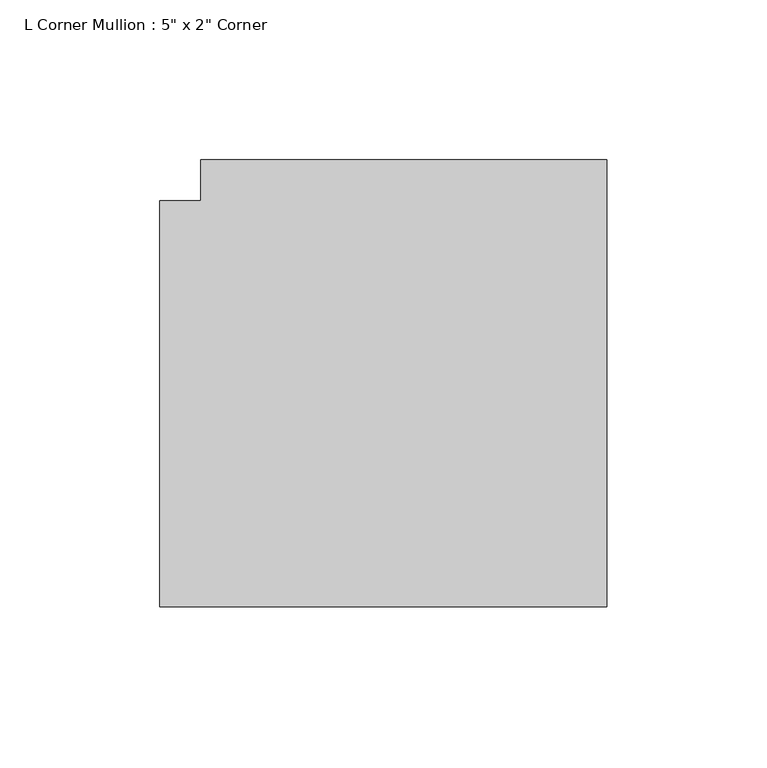
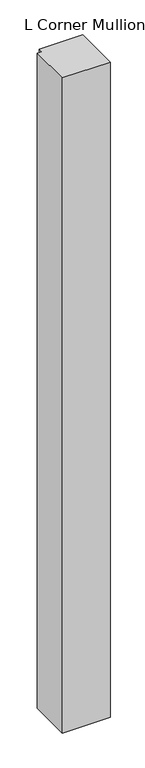
"""IFC4 building model written with IfcOpenShell, lengths in millimetres: member geometry."""

from ifc_helpers import new_model, si_unit, frame, origin, place, context, project, spatial, polyline, outline, extrude, source, transform, mapped, element, save


def member_8e92f094(model_context):
    return source(origin(), model_context, "Body", "SweptSolid", [
        extrude(outline(polyline([(63.5, 76.2), (63.5, -63.5), (-76.2, -63.5), (-76.2, 63.5), (-63.5, 63.5), (-63.5, 76.2), (63.5, 76.2)])), frame((0.0, 0.0, -2032.0), z_axis=(0.0, 0.0, 1.0), x_axis=(1.0, 0.0, 0.0)), (0.0, 0.0, 1.0), 2032.0),
    ])


if __name__ == "__main__":
    model = new_model("IFC4")
    model_context = context("Model", 3, world=origin())
    ifc_project = project(units=[si_unit("LENGTHUNIT", "METRE", prefix="MILLI")], contexts=[model_context])
    site = spatial("IfcSite", under=ifc_project)
    building = spatial("IfcBuilding", under=site)
    placement = place(None, origin())
    member_shape = member_8e92f094(model_context)
    element("IfcMember", 1, ObjectType="L Corner Mullion : 5\" x 2\" Corner", at=placement, inside=building, context=model_context, shape_type="MappedRepresentation", body=[
        mapped(member_shape, transform((0.0, 0.0, 0.0), x_axis=(1.0, 0.0, 0.0), y_axis=(0.0, 1.0, 0.0), z_axis=(0.0, 0.0, 1.0))),
    ])
    save(model, "model.ifc")

# Revit data of these elements
# Type "L Corner Mullion : 5\" x 2\" Corner"
#   built-in parameter 1007355 = 0.25 (stored number, unit not read)
#   built-in parameter 1007354 = 0.25 (stored number, unit not read)
#   built-in parameter 1007304 = 0.416667 (stored number, unit not read)
# Element 1 (IfcMember, "L Corner Mullion : 5\" x 2\" Corner")
#   Materials on its faces: "Metal - Aluminum"
# Materials
#   "Metal - Aluminum": class "Metal", colour RGB 109 108 108, transparency 0
